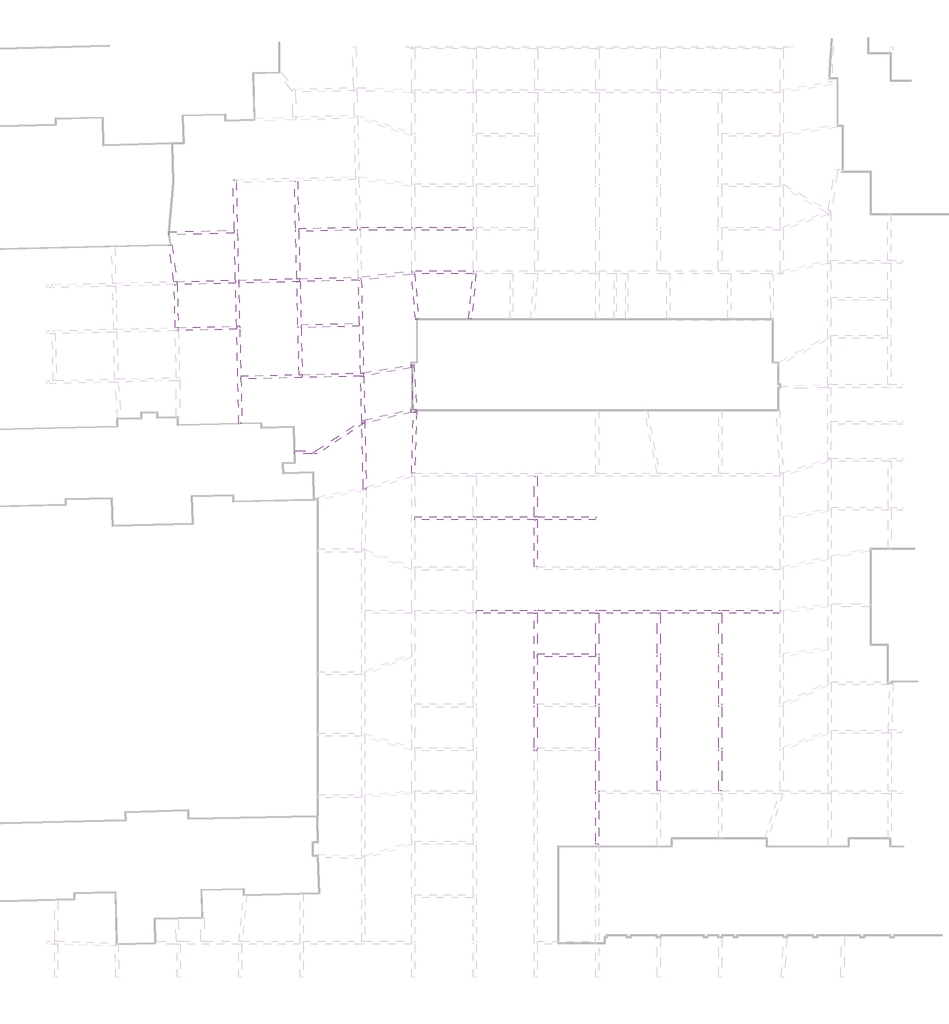
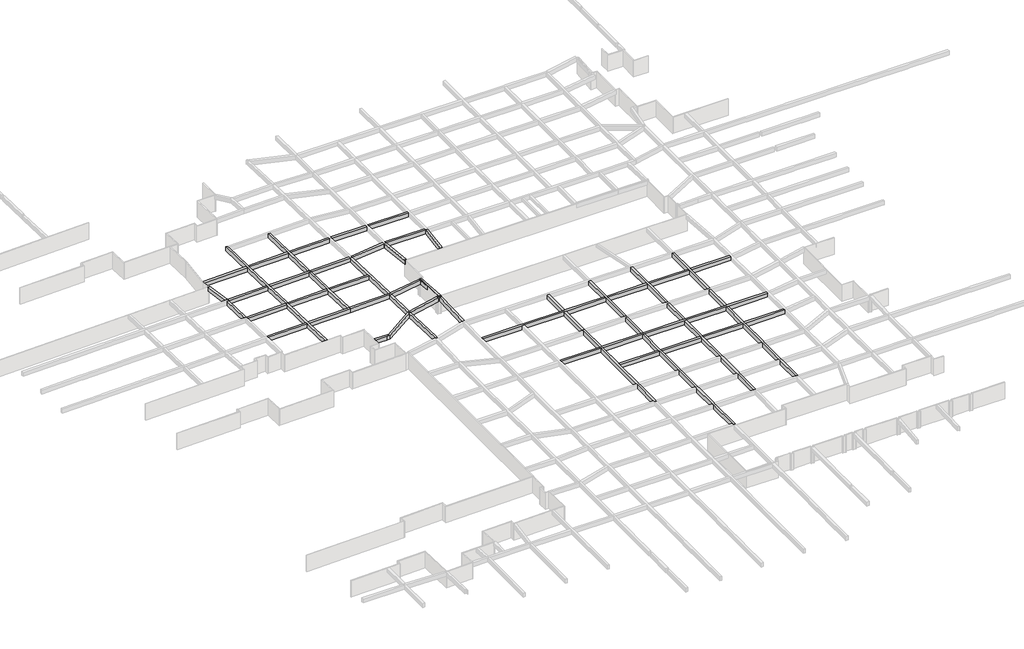
# One storey, part 11 of 20: 39 beams.
"""IFC4 building model written with IfcOpenShell, lengths in millimetres."""

from ifc_helpers import new_model, si_unit, frame, origin, place, context, project, spatial, polyline, outline, extrude, faceted_brep, element, save

model = new_model("IFC4")

# Units and contexts
model_context = context("Model", 3, world=origin())
ifc_project = project(units=[si_unit("LENGTHUNIT", "METRE", prefix="MILLI")], contexts=[model_context])

# Site, building, storey
site = spatial("IfcSite", under=ifc_project)
building = spatial("IfcBuilding", under=site)
storey = spatial("IfcBuildingStorey", under=building, Name="户型图", Elevation=0.0)

# Beams
placement = place(None, origin())
element("IfcBeam", 1, ObjectType="混凝土 - 矩形梁 : KL_beam", at=placement, inside=storey, context=model_context, shape_type="SweptSolid", body=[
    extrude(outline(polyline([(54450.0, 125765.1975441), (54450.0, 125365.1975441), (47756.2911881, 125365.1975441), (47746.6524387, 125765.1975441), (54450.0, 125765.1975441)])), frame((0.0, 0.0, 2500.0), z_axis=(0.0, 0.0, 1.0), x_axis=(1.0, 0.0, 0.0)), (0.0, 0.0, 1.0), 800.0),
])
element("IfcBeam", 2, ObjectType="混凝土 - 矩形梁 : KL_beam", at=placement, inside=storey, context=model_context, shape_type="SweptSolid", body=[
    extrude(outline(polyline([(62450.0, 125765.1975441), (62450.0, 125365.1975441), (54850.0, 125365.1975441), (54850.0, 125765.1975441), (62450.0, 125765.1975441)])), frame((0.0, 0.0, 2500.0), z_axis=(0.0, 0.0, 1.0), x_axis=(1.0, 0.0, 0.0)), (0.0, 0.0, 1.0), 800.0),
])
element("IfcBeam", 3, ObjectType="混凝土 - 矩形梁 : KL_beam", at=placement, inside=storey, context=model_context, shape_type="SweptSolid", body=[
    extrude(outline(polyline([(54450.0, 119664.8886593), (47912.3274647, 118889.8231887), (47902.648865, 119291.4769437), (54450.0, 120067.6898484), (54450.0, 119664.8886593)])), frame((0.0, 0.0, 2500.0), z_axis=(0.0, 0.0, 1.0), x_axis=(1.0, 0.0, 0.0)), (0.0, 0.0, 1.0), 800.0),
])
element("IfcBeam", 4, ObjectType="混凝土 - 矩形梁 : KL_beam", at=placement, inside=storey, context=model_context, shape_type="Brep", body=[
    faceted_brep([(62450.0, 119690.0, 3300.0), (62450.0, 120090.0, 3300.0), (54850.0, 120090.0, 3300.0), (54850.0, 119712.3101516, 3300.0), (54661.8140065, 119690.0, 3300.0), (54867.3687974, 119690.0, 3300.0), (62430.2407958, 119690.0, 3300.0), (62450.0, 119690.0, 2500.0), (54661.8140065, 119690.0, 2500.0), (54867.3687974, 119690.0, 2500.0), (62430.2407958, 119690.0, 2500.0), (62450.0, 120090.0, 2500.0), (54850.0, 119712.3101516, 2500.0), (54850.0, 120090.0, 2500.0)], [[[0, 1, 2, 3, 4, 5, 6]], [[7, 0, 6, 5, 4, 8, 9, 10]], [[11, 7, 10, 9, 8, 12, 13]], [[1, 11, 13, 2]], [[1, 0, 7, 11]], [[12, 3, 2, 13]], [[3, 12, 8, 4]]]),
])
element("IfcBeam", 5, ObjectType="混凝土 - 矩形梁 : KL_beam", at=placement, inside=storey, context=model_context, shape_type="Brep", body=[
    faceted_brep([(102445.0, 75460.0, 3300.0), (102445.0, 75860.0, 3300.0), (94850.0, 75860.0, 3300.0), (94450.0, 75860.0, 3300.0), (86850.0, 75860.0, 3300.0), (86450.0, 75860.0, 3300.0), (78850.0, 75860.0, 3300.0), (78450.0, 75860.0, 3300.0), (70850.0, 75860.0, 3300.0), (70450.0, 75860.0, 3300.0), (62850.0, 75860.0, 3300.0), (62850.0, 75460.0, 3300.0), (70450.0, 75460.0, 3300.0), (70850.0, 75460.0, 3300.0), (78450.0, 75460.0, 3300.0), (78850.0, 75460.0, 3300.0), (86450.0, 75460.0, 3300.0), (86850.0, 75460.0, 3300.0), (94450.0, 75460.0, 3300.0), (94850.0, 75460.0, 3300.0), (102445.0, 75460.0, 2500.0), (62850.0, 75460.0, 2500.0), (70450.0, 75460.0, 2500.0), (70850.0, 75460.0, 2500.0), (78450.0, 75460.0, 2500.0), (78850.0, 75460.0, 2500.0), (86450.0, 75460.0, 2500.0), (86850.0, 75460.0, 2500.0), (94450.0, 75460.0, 2500.0), (94850.0, 75460.0, 2500.0), (102445.0, 75860.0, 2500.0), (62850.0, 75860.0, 2500.0), (70450.0, 75860.0, 2500.0), (70850.0, 75860.0, 2500.0), (78450.0, 75860.0, 2500.0), (78850.0, 75860.0, 2500.0), (86450.0, 75860.0, 2500.0), (86850.0, 75860.0, 2500.0), (94450.0, 75860.0, 2500.0), (94850.0, 75860.0, 2500.0)], [[[0, 1, 2, 3, 4, 5, 6, 7, 8, 9, 10, 11, 12, 13, 14, 15, 16, 17, 18, 19]], [[20, 0, 19, 18, 17, 16, 15, 14, 13, 12, 11, 21, 22, 23, 24, 25, 26, 27, 28, 29]], [[30, 20, 29, 28, 27, 26, 25, 24, 23, 22, 21, 31, 32, 33, 34, 35, 36, 37, 38, 39]], [[1, 30, 39, 38, 37, 36, 35, 34, 33, 32, 31, 10, 9, 8, 7, 6, 5, 4, 3, 2]], [[1, 0, 20, 30]], [[11, 10, 31, 21]]]),
])
element("IfcBeam", 6, ObjectType="混凝土 - 矩形梁 : KL_beam", at=placement, inside=storey, context=model_context, shape_type="Brep", body=[
    faceted_brep([(70450.0, 57560.0, 3300.0), (70850.0, 57560.0, 3300.0), (70850.0, 57960.0, 3300.0), (70850.0, 63283.0, 3300.0), (70850.0, 63683.0, 3300.0), (70850.0, 69810.0, 3300.0), (70850.0, 70210.0, 3300.0), (70850.0, 75460.0, 3300.0), (70450.0, 75460.0, 3300.0), (70450.0, 63660.0, 3300.0), (70450.0, 63260.0, 3300.0), (70450.0, 57960.0, 3300.0), (70450.0, 57560.0, 2500.0), (70450.0, 75460.0, 2500.0), (70450.0, 63660.0, 2500.0), (70450.0, 63260.0, 2500.0), (70450.0, 57960.0, 2500.0), (70850.0, 57560.0, 2500.0), (70850.0, 75460.0, 2500.0), (70850.0, 70210.0, 2500.0), (70850.0, 69810.0, 2500.0), (70850.0, 63683.0, 2500.0), (70850.0, 63283.0, 2500.0), (70850.0, 57960.0, 2500.0)], [[[0, 1, 2, 3, 4, 5, 6, 7, 8, 9, 10, 11]], [[12, 0, 11, 10, 9, 8, 13, 14, 15, 16]], [[17, 12, 16, 15, 14, 13, 18, 19, 20, 21, 22, 23]], [[1, 17, 23, 22, 21, 20, 19, 18, 7, 6, 5, 4, 3, 2]], [[8, 7, 18, 13]], [[1, 0, 12, 17]]]),
    faceted_brep([(70850.0, 75860.0, 3300.0), (70450.0, 75860.0, 3300.0), (70450.0, 75860.0, 2500.0), (70850.0, 75860.0, 2500.0), (70850.0, 81560.0, 3300.0), (70450.0, 81560.0, 3300.0), (70450.0, 81510.0, 3300.0), (70450.0, 81110.0, 3300.0), (70850.0, 81160.0, 3300.0), (70450.0, 81560.0, 2500.0), (70450.0, 81510.0, 2500.0), (70450.0, 81110.0, 2500.0), (70850.0, 81560.0, 2500.0), (70850.0, 81160.0, 2500.0)], [[[0, 1, 2, 3]], [[4, 5, 6, 7, 1, 0, 8]], [[5, 9, 10, 11, 2, 1, 7, 6]], [[9, 12, 13, 3, 2, 11, 10]], [[12, 4, 8, 0, 3, 13]], [[5, 4, 12, 9]]]),
])
element("IfcBeam", 7, ObjectType="混凝土 - 矩形梁 : KL_beam", at=placement, inside=storey, context=model_context, shape_type="Brep", body=[
    faceted_brep([(78450.0, 81560.0, 3300.0), (78850.0, 81560.0, 3300.0), (78850.0, 87660.0, 3300.0), (78850.0, 88060.0, 3300.0), (78850.0, 93310.0, 3300.0), (78450.0, 93310.0, 3300.0), (78450.0, 88060.0, 3300.0), (78450.0, 87660.0, 3300.0), (78450.0, 81560.0, 2500.0), (78450.0, 93310.0, 2500.0), (78450.0, 88060.0, 2500.0), (78450.0, 87660.0, 2500.0), (78850.0, 81560.0, 2500.0), (78850.0, 93310.0, 2500.0), (78850.0, 88060.0, 2500.0), (78850.0, 87660.0, 2500.0)], [[[0, 1, 2, 3, 4, 5, 6, 7]], [[8, 0, 7, 6, 5, 9, 10, 11]], [[12, 8, 11, 10, 9, 13, 14, 15]], [[1, 12, 15, 14, 13, 4, 3, 2]], [[1, 0, 8, 12]], [[5, 4, 13, 9]]]),
    faceted_brep([(78450.0, 75460.0, 3300.0), (78850.0, 75460.0, 3300.0), (78850.0, 75460.0, 2500.0), (78450.0, 75460.0, 2500.0), (78450.0, 70210.0, 3300.0), (78450.0, 69810.0, 3300.0), (78450.0, 63683.0, 3300.0), (78450.0, 63283.0, 3300.0), (78450.0, 57960.0, 3300.0), (78450.0, 57560.0, 3300.0), (78450.0, 52365.0, 3300.0), (78450.0, 51965.0, 3300.0), (78450.0, 45760.0, 3300.0), (78450.0, 45360.0, 3300.0), (78850.0, 45360.0, 3300.0), (78850.0, 51965.0, 3300.0), (78850.0, 52365.0, 3300.0), (78850.0, 57560.0, 3300.0), (78850.0, 57960.0, 3300.0), (78850.0, 63283.0, 3300.0), (78850.0, 63683.0, 3300.0), (78850.0, 69810.0, 3300.0), (78850.0, 70210.0, 3300.0), (78450.0, 70210.0, 2500.0), (78450.0, 69810.0, 2500.0), (78450.0, 63683.0, 2500.0), (78450.0, 63283.0, 2500.0), (78450.0, 57960.0, 2500.0), (78450.0, 57560.0, 2500.0), (78450.0, 52365.0, 2500.0), (78450.0, 51965.0, 2500.0), (78450.0, 45760.0, 2500.0), (78450.0, 45360.0, 2500.0), (78850.0, 70210.0, 2500.0), (78850.0, 69810.0, 2500.0), (78850.0, 63683.0, 2500.0), (78850.0, 63283.0, 2500.0), (78850.0, 57960.0, 2500.0), (78850.0, 57560.0, 2500.0), (78850.0, 52365.0, 2500.0), (78850.0, 51965.0, 2500.0), (78850.0, 45360.0, 2500.0)], [[[0, 1, 2, 3]], [[1, 0, 4, 5, 6, 7, 8, 9, 10, 11, 12, 13, 14, 15, 16, 17, 18, 19, 20, 21, 22]], [[0, 3, 23, 24, 25, 26, 27, 28, 29, 30, 31, 32, 13, 12, 11, 10, 9, 8, 7, 6, 5, 4]], [[3, 2, 33, 34, 35, 36, 37, 38, 39, 40, 41, 32, 31, 30, 29, 28, 27, 26, 25, 24, 23]], [[2, 1, 22, 21, 20, 19, 18, 17, 16, 15, 14, 41, 40, 39, 38, 37, 36, 35, 34, 33]], [[14, 13, 32, 41]]]),
    faceted_brep([(78850.0, 75860.0, 3300.0), (78450.0, 75860.0, 3300.0), (78450.0, 75860.0, 2500.0), (78850.0, 75860.0, 2500.0), (78450.0, 81160.0, 3300.0), (78850.0, 81160.0, 3300.0), (78850.0, 81160.0, 2500.0), (78450.0, 81160.0, 2500.0)], [[[0, 1, 2, 3]], [[4, 5, 6, 7]], [[1, 0, 5, 4]], [[2, 1, 4, 7]], [[3, 2, 7, 6]], [[0, 3, 6, 5]]]),
])
element("IfcBeam", 8, ObjectType="混凝土 - 矩形梁 : KL_beam", at=placement, inside=storey, context=model_context, shape_type="Brep", body=[
    faceted_brep([(86450.0, 81560.0, 3300.0), (86850.0, 81560.0, 3300.0), (86850.0, 87660.0, 3300.0), (86850.0, 88060.0, 3300.0), (86850.0, 93310.0, 3300.0), (86450.0, 93310.0, 3300.0), (86450.0, 88060.0, 3300.0), (86450.0, 87660.0, 3300.0), (86450.0, 81560.0, 2500.0), (86450.0, 93310.0, 2500.0), (86450.0, 88060.0, 2500.0), (86450.0, 87660.0, 2500.0), (86850.0, 81560.0, 2500.0), (86850.0, 93310.0, 2500.0), (86850.0, 88060.0, 2500.0), (86850.0, 87660.0, 2500.0)], [[[0, 1, 2, 3, 4, 5, 6, 7]], [[8, 0, 7, 6, 5, 9, 10, 11]], [[12, 8, 11, 10, 9, 13, 14, 15]], [[1, 12, 15, 14, 13, 4, 3, 2]], [[1, 0, 8, 12]], [[5, 4, 13, 9]]]),
    faceted_brep([(86450.0, 75460.0, 3300.0), (86850.0, 75460.0, 3300.0), (86850.0, 75460.0, 2500.0), (86450.0, 75460.0, 2500.0), (86450.0, 70210.0, 3300.0), (86450.0, 69810.0, 3300.0), (86450.0, 63683.0, 3300.0), (86450.0, 63283.0, 3300.0), (86450.0, 57960.0, 3300.0), (86450.0, 57560.0, 3300.0), (86450.0, 52365.0, 3300.0), (86850.0, 52365.0, 3300.0), (86850.0, 57560.0, 3300.0), (86850.0, 57960.0, 3300.0), (86850.0, 63283.0, 3300.0), (86850.0, 63683.0, 3300.0), (86850.0, 69810.0, 3300.0), (86850.0, 70210.0, 3300.0), (86450.0, 70210.0, 2500.0), (86450.0, 69810.0, 2500.0), (86450.0, 63683.0, 2500.0), (86450.0, 63283.0, 2500.0), (86450.0, 57960.0, 2500.0), (86450.0, 57560.0, 2500.0), (86450.0, 52365.0, 2500.0), (86850.0, 70210.0, 2500.0), (86850.0, 69810.0, 2500.0), (86850.0, 63683.0, 2500.0), (86850.0, 63283.0, 2500.0), (86850.0, 57960.0, 2500.0), (86850.0, 57560.0, 2500.0), (86850.0, 52365.0, 2500.0)], [[[0, 1, 2, 3]], [[1, 0, 4, 5, 6, 7, 8, 9, 10, 11, 12, 13, 14, 15, 16, 17]], [[0, 3, 18, 19, 20, 21, 22, 23, 24, 10, 9, 8, 7, 6, 5, 4]], [[3, 2, 25, 26, 27, 28, 29, 30, 31, 24, 23, 22, 21, 20, 19, 18]], [[2, 1, 17, 16, 15, 14, 13, 12, 11, 31, 30, 29, 28, 27, 26, 25]], [[11, 10, 24, 31]]]),
    faceted_brep([(86850.0, 75860.0, 3300.0), (86450.0, 75860.0, 3300.0), (86450.0, 75860.0, 2500.0), (86850.0, 75860.0, 2500.0), (86450.0, 81160.0, 3300.0), (86850.0, 81160.0, 3300.0), (86850.0, 81160.0, 2500.0), (86450.0, 81160.0, 2500.0)], [[[0, 1, 2, 3]], [[4, 5, 6, 7]], [[1, 0, 5, 4]], [[2, 1, 4, 7]], [[3, 2, 7, 6]], [[0, 3, 6, 5]]]),
])
element("IfcBeam", 9, ObjectType="混凝土 - 矩形梁 : KL_beam", at=placement, inside=storey, context=model_context, shape_type="Brep", body=[
    faceted_brep([(94850.0, 75460.0, 3300.0), (94450.0, 75460.0, 3300.0), (94450.0, 70210.0, 3300.0), (94450.0, 69810.0, 3300.0), (94450.0, 63683.0, 3300.0), (94450.0, 63283.0, 3300.0), (94450.0, 57960.0, 3300.0), (94450.0, 57560.0, 3300.0), (94450.0, 52365.0, 3300.0), (94850.0, 52365.0, 3300.0), (94850.0, 57560.0, 3300.0), (94850.0, 57960.0, 3300.0), (94850.0, 63283.0, 3300.0), (94850.0, 63683.0, 3300.0), (94850.0, 69810.0, 3300.0), (94850.0, 70210.0, 3300.0), (94850.0, 75460.0, 2500.0), (94850.0, 52365.0, 2500.0), (94850.0, 57560.0, 2500.0), (94850.0, 57960.0, 2500.0), (94850.0, 63283.0, 2500.0), (94850.0, 63683.0, 2500.0), (94850.0, 69810.0, 2500.0), (94850.0, 70210.0, 2500.0), (94450.0, 75460.0, 2500.0), (94450.0, 52365.0, 2500.0), (94450.0, 57560.0, 2500.0), (94450.0, 57960.0, 2500.0), (94450.0, 63283.0, 2500.0), (94450.0, 63683.0, 2500.0), (94450.0, 69810.0, 2500.0), (94450.0, 70210.0, 2500.0)], [[[0, 1, 2, 3, 4, 5, 6, 7, 8, 9, 10, 11, 12, 13, 14, 15]], [[16, 0, 15, 14, 13, 12, 11, 10, 9, 17, 18, 19, 20, 21, 22, 23]], [[24, 16, 23, 22, 21, 20, 19, 18, 17, 25, 26, 27, 28, 29, 30, 31]], [[1, 24, 31, 30, 29, 28, 27, 26, 25, 8, 7, 6, 5, 4, 3, 2]], [[1, 0, 16, 24]], [[9, 8, 25, 17]]]),
    faceted_brep([(94850.0, 75860.0, 3300.0), (94450.0, 75860.0, 3300.0), (94450.0, 75860.0, 2500.0), (94850.0, 75860.0, 2500.0), (94450.0, 81160.0, 3300.0), (94850.0, 81160.0, 3300.0), (94850.0, 81160.0, 2500.0), (94450.0, 81160.0, 2500.0)], [[[0, 1, 2, 3]], [[4, 5, 6, 7]], [[1, 0, 5, 4]], [[0, 3, 6, 5]], [[3, 2, 7, 6]], [[2, 1, 4, 7]]]),
    faceted_brep([(94450.0, 81560.0, 3300.0), (94850.0, 81560.0, 3300.0), (94850.0, 87660.0, 3300.0), (94850.0, 88060.0, 3300.0), (94850.0, 93310.0, 3300.0), (94450.0, 93310.0, 3300.0), (94450.0, 88060.0, 3300.0), (94450.0, 87660.0, 3300.0), (94850.0, 81560.0, 2500.0), (94850.0, 87660.0, 2500.0), (94850.0, 88060.0, 2500.0), (94850.0, 93310.0, 2500.0), (94450.0, 81560.0, 2500.0), (94450.0, 87660.0, 2500.0), (94450.0, 88060.0, 2500.0), (94450.0, 93310.0, 2500.0)], [[[0, 1, 2, 3, 4, 5, 6, 7]], [[1, 8, 9, 10, 11, 4, 3, 2]], [[8, 12, 13, 14, 15, 11, 10, 9]], [[12, 0, 7, 6, 5, 15, 14, 13]], [[1, 0, 12, 8]], [[5, 4, 11, 15]]]),
])
element("IfcBeam", 10, ObjectType="混凝土 - 矩形梁 : KL_beam", at=placement, inside=storey, context=model_context, shape_type="Brep", body=[
    faceted_brep([(78450.0, 87660.0, 3300.0), (78450.0, 88060.0, 3300.0), (70850.0, 88060.0, 3300.0), (70450.0, 88060.0, 3300.0), (62850.0, 88060.0, 3300.0), (62450.0, 88060.0, 3300.0), (54850.0, 88060.0, 3300.0), (54850.0, 87660.0, 3300.0), (62450.0, 87660.0, 3300.0), (62850.0, 87660.0, 3300.0), (70450.0, 87660.0, 3300.0), (70850.0, 87660.0, 3300.0), (78450.0, 87660.0, 2500.0), (54850.0, 87660.0, 2500.0), (62450.0, 87660.0, 2500.0), (62850.0, 87660.0, 2500.0), (70450.0, 87660.0, 2500.0), (70850.0, 87660.0, 2500.0), (78450.0, 88060.0, 2500.0), (54850.0, 88060.0, 2500.0), (62450.0, 88060.0, 2500.0), (62850.0, 88060.0, 2500.0), (70450.0, 88060.0, 2500.0), (70850.0, 88060.0, 2500.0)], [[[0, 1, 2, 3, 4, 5, 6, 7, 8, 9, 10, 11]], [[12, 0, 11, 10, 9, 8, 7, 13, 14, 15, 16, 17]], [[18, 12, 17, 16, 15, 14, 13, 19, 20, 21, 22, 23]], [[1, 18, 23, 22, 21, 20, 19, 6, 5, 4, 3, 2]], [[1, 0, 12, 18]], [[7, 6, 19, 13]]]),
    faceted_brep([(102445.0, 88060.0, 3300.0), (102445.0, 87660.0, 3300.0), (102445.0, 87660.0, 2500.0), (102445.0, 88060.0, 2500.0), (94850.0, 87660.0, 3300.0), (94850.0, 88060.0, 3300.0), (94850.0, 88060.0, 2500.0), (94850.0, 87660.0, 2500.0)], [[[0, 1, 2, 3]], [[4, 5, 6, 7]], [[1, 0, 5, 4]], [[2, 1, 4, 7]], [[3, 2, 7, 6]], [[0, 3, 6, 5]]]),
    faceted_brep([(78850.0, 87660.0, 3300.0), (78850.0, 88060.0, 3300.0), (78850.0, 88060.0, 2500.0), (78850.0, 87660.0, 2500.0), (86450.0, 88060.0, 3300.0), (86450.0, 87660.0, 3300.0), (86450.0, 87660.0, 2500.0), (86450.0, 88060.0, 2500.0)], [[[0, 1, 2, 3]], [[4, 5, 6, 7]], [[1, 0, 5, 4]], [[0, 3, 6, 5]], [[3, 2, 7, 6]], [[2, 1, 4, 7]]]),
    faceted_brep([(86850.0, 88060.0, 3300.0), (86850.0, 87660.0, 3300.0), (94450.0, 87660.0, 3300.0), (94450.0, 88060.0, 3300.0), (86850.0, 87660.0, 2500.0), (94450.0, 87660.0, 2500.0), (86850.0, 88060.0, 2500.0), (94450.0, 88060.0, 2500.0)], [[[0, 1, 2, 3]], [[1, 4, 5, 2]], [[4, 6, 7, 5]], [[6, 0, 3, 7]], [[1, 0, 6, 4]], [[3, 2, 5, 7]]]),
])
element("IfcBeam", 11, ObjectType="混凝土 - 矩形梁 : KL_beam", at=placement, inside=storey, context=model_context, shape_type="SweptSolid", body=[
    extrude(outline(polyline([(102445.0, 70210.0), (102445.0, 69810.0), (94850.0, 69810.0), (94850.0, 70210.0), (102445.0, 70210.0)])), frame((0.0, 0.0, 2500.0), z_axis=(0.0, 0.0, 1.0), x_axis=(1.0, 0.0, 0.0)), (0.0, 0.0, 1.0), 800.0),
    extrude(outline(polyline([(70850.0, 69810.0), (70850.0, 70210.0), (78450.0, 70210.0), (78450.0, 69810.0), (70850.0, 69810.0)])), frame((0.0, 0.0, 2500.0), z_axis=(0.0, 0.0, 1.0), x_axis=(1.0, 0.0, 0.0)), (0.0, 0.0, 1.0), 800.0),
    extrude(outline(polyline([(78850.0, 69810.0), (78850.0, 70210.0), (86450.0, 70210.0), (86450.0, 69810.0), (78850.0, 69810.0)])), frame((0.0, 0.0, 2500.0), z_axis=(0.0, 0.0, 1.0), x_axis=(1.0, 0.0, 0.0)), (0.0, 0.0, 1.0), 800.0),
    extrude(outline(polyline([(86850.0, 69810.0), (86850.0, 70210.0), (94450.0, 70210.0), (94450.0, 69810.0), (86850.0, 69810.0)])), frame((0.0, 0.0, 2500.0), z_axis=(0.0, 0.0, 1.0), x_axis=(1.0, 0.0, 0.0)), (0.0, 0.0, 1.0), 800.0),
])
element("IfcBeam", 12, ObjectType="混凝土 - 矩形梁 : KL_beam", at=placement, inside=storey, context=model_context, shape_type="SweptSolid", body=[
    extrude(outline(polyline([(70450.0, 93310.0), (70850.0, 93310.0), (70850.0, 88060.0), (70450.0, 88060.0), (70450.0, 93310.0)])), frame((0.0, 0.0, 2500.0), z_axis=(0.0, 0.0, 1.0), x_axis=(1.0, 0.0, 0.0)), (0.0, 0.0, 1.0), 800.0),
])
element("IfcBeam", 13, ObjectType="混凝土 - 矩形梁 : KL_beam", at=placement, inside=storey, context=model_context, shape_type="SweptSolid", body=[
    extrude(outline(polyline([(70850.0, 81560.0), (70450.0, 81560.0), (70450.0, 87660.0), (70850.0, 87660.0), (70850.0, 81560.0)])), frame((0.0, 0.0, 2500.0), z_axis=(0.0, 0.0, 1.0), x_axis=(1.0, 0.0, 0.0)), (0.0, 0.0, 1.0), 800.0),
])
element("IfcBeam", 14, ObjectType="混凝土 - 矩形梁 : KL_beam", at=placement, inside=storey, context=model_context, shape_type="Brep", body=[
    faceted_brep([(61879.8710047, 113857.0, 3300.0), (62281.6476136, 113857.0, 3300.0), (62832.0174047, 119690.0, 3300.0), (62450.0, 119690.0, 3300.0), (62430.2407958, 119690.0, 3300.0), (61879.8710047, 113857.0, 2500.0), (62430.2407958, 119690.0, 2500.0), (62281.6476136, 113857.0, 2500.0), (62450.0, 119690.0, 2500.0), (62832.0174047, 119690.0, 2500.0)], [[[0, 1, 2, 3, 4]], [[5, 0, 4, 6]], [[7, 5, 6, 8, 9]], [[1, 7, 9, 2]], [[1, 0, 5, 7]], [[2, 9, 8, 6, 4, 3]]]),
])
element("IfcBeam", 15, ObjectType="混凝土 - 矩形梁 : KL_beam", at=placement, inside=storey, context=model_context, shape_type="SweptSolid", body=[
    extrude(outline(polyline([(55098.0, 113737.0), (54962.3085372, 113737.0), (54467.8976834, 119667.0104964), (54661.8140065, 119690.0), (54867.3687974, 119690.0), (55353.6914628, 113857.0), (55098.0, 113857.0), (55098.0, 113737.0)])), frame((0.0, 0.0, 2500.0), z_axis=(0.0, 0.0, 1.0), x_axis=(1.0, 0.0, 0.0)), (0.0, 0.0, 1.0), 800.0),
])
element("IfcBeam", 16, ObjectType="混凝土 - 矩形梁 : KL_beam", at=placement, inside=storey, context=model_context, shape_type="SweptSolid", body=[
    extrude(outline(polyline([(22839.9092142, 123427.099828), (23236.2427496, 123481.1343421), (23889.0031982, 118693.2527351), (23486.6252708, 118683.5527596), (22839.9092142, 123427.099828)])), frame((0.0, 0.0, 2500.0), z_axis=(0.0, 0.0, 1.0), x_axis=(1.0, 0.0, 0.0)), (0.0, 0.0, 1.0), 800.0),
])
element("IfcBeam", 17, ObjectType="混凝土 - 矩形梁 : KL_beam", at=placement, inside=storey, context=model_context, shape_type="Brep", body=[
    faceted_brep([(23889.0031982, 118693.2527351, 3300.0), (23898.6430493, 118293.3689104, 3300.0), (23540.9968018, 118284.7472649, 3300.0), (23519.8781337, 118284.238165, 3300.0), (23654.8569706, 112685.136784, 3300.0), (24054.7407895, 112694.7768761, 3300.0), (23919.7618713, 118293.8816298, 3300.0), (23910.1218663, 118693.761835, 3300.0), (23519.8781337, 118284.238165, 2500.0), (23654.8569706, 112685.136784, 2500.0), (23898.6430493, 118293.3689104, 2500.0), (23889.0031982, 118693.2527351, 2500.0), (23910.1218663, 118693.761835, 2500.0), (23919.7618713, 118293.8816298, 2500.0), (24054.7407895, 112694.7768761, 2500.0), (23540.9968018, 118284.7472649, 2500.0)], [[[0, 1, 2, 3, 4, 5, 6, 7]], [[3, 8, 9, 4]], [[10, 11, 12, 13, 14, 9, 8, 15]], [[12, 7, 6, 5, 14, 13]], [[11, 0, 7, 12]], [[1, 10, 15, 8, 3, 2]], [[10, 1, 0, 11]], [[5, 4, 9, 14]]]),
])
element("IfcBeam", 18, ObjectType="混凝土 - 矩形梁 : KL_beam", at=placement, inside=storey, context=model_context, shape_type="Brep", body=[
    faceted_brep([(32052.1182859, 112886.7653645, 3300.0), (31652.2346355, 112877.1182859, 3300.0), (31661.8588222, 112478.1835343, 3300.0), (31956.7693302, 100253.7688116, 3300.0), (32356.6529807, 100263.4158903, 3300.0), (32218.5158115, 105989.3768117, 3300.0), (32208.8687328, 106389.2604627, 3300.0), (32061.7653645, 112486.8817141, 3300.0), (31652.2346355, 112877.1182859, 2500.0), (31661.8588222, 112478.1835343, 2500.0), (31956.7693302, 100253.7688116, 2500.0), (32052.1182859, 112886.7653645, 2500.0), (32061.7653645, 112486.8817141, 2500.0), (32208.8687328, 106389.2604627, 2500.0), (32218.5158115, 105989.3768117, 2500.0), (32356.6529807, 100263.4158903, 2500.0)], [[[0, 1, 2, 3, 4, 5, 6, 7]], [[1, 8, 9, 10, 3, 2]], [[8, 11, 12, 13, 14, 15, 10, 9]], [[11, 0, 7, 6, 5, 4, 15, 14, 13, 12]], [[4, 3, 10, 15]], [[1, 0, 11, 8]]]),
])
element("IfcBeam", 19, ObjectType="混凝土 - 矩形梁 : KL_beam", at=placement, inside=storey, context=model_context, shape_type="Brep", body=[
    faceted_brep([(24216.2679247, 105994.416832, 3300.0), (24221.0300595, 105796.8771597, 3300.0), (31818.6316338, 105979.7515911, 3300.0), (31808.9845551, 106379.6352421, 3300.0), (24216.2679247, 106196.8783914, 3300.0), (24221.0300595, 105796.8771597, 2500.0), (31818.6316338, 105979.7515911, 2500.0), (24216.2679247, 105994.416832, 2500.0), (24216.2679247, 106196.8783914, 2500.0), (31808.9845551, 106379.6352421, 2500.0)], [[[0, 1, 2, 3, 4]], [[1, 5, 6, 2]], [[5, 7, 8, 9, 6]], [[8, 4, 3, 9]], [[5, 1, 0, 7]], [[0, 4, 8, 7]], [[3, 2, 6, 9]]]),
    faceted_brep([(32218.5158115, 105989.3768117, 3300.0), (32208.8687328, 106389.2604627, 3300.0), (32208.8687328, 106389.2604627, 2500.0), (32218.5158115, 105989.3768117, 2500.0), (40215.5578613, 106181.8657839, 3300.0), (40205.9326406, 106581.749961, 3300.0), (39806.0484635, 106572.1247404, 3300.0), (40215.5578613, 106181.8657839, 2500.0), (40205.9326406, 106581.749961, 2500.0), (39806.0484635, 106572.1247404, 2500.0)], [[[0, 1, 2, 3]], [[4, 5, 6, 1, 0]], [[7, 4, 0, 3]], [[8, 7, 3, 2, 9]], [[5, 8, 9, 2, 1, 6]], [[5, 4, 7, 8]]]),
])
element("IfcBeam", 20, ObjectType="混凝土 - 矩形梁 : KL_beam", at=placement, inside=storey, context=model_context, shape_type="Brep", body=[
    faceted_brep([(40205.9323475, 106581.7621411, 3300.0), (40215.5575681, 106181.8779632, 3300.0), (47814.3531628, 106365.2447486, 3300.0), (48028.6784416, 106370.4166389, 3300.0), (48214.331784, 106374.8966458, 3300.0), (48213.6881872, 106401.5675651, 3300.0), (48204.68218, 106774.7802353, 3300.0), (47804.7985905, 106765.1306313, 3300.0), (40215.5575681, 106181.8779632, 2500.0), (47814.3531628, 106365.2447486, 2500.0), (48028.6784416, 106370.4166389, 2500.0), (48214.331784, 106374.8966458, 2500.0), (40205.9323475, 106581.7621411, 2500.0), (47804.7985905, 106765.1306313, 2500.0), (48204.68218, 106774.7802353, 2500.0), (48213.6881872, 106401.5675651, 2500.0)], [[[0, 1, 2, 3, 4, 5, 6, 7]], [[1, 8, 9, 10, 11, 4, 3, 2]], [[8, 12, 13, 14, 15, 11, 10, 9]], [[12, 0, 7, 6, 14, 13]], [[1, 0, 12, 8]], [[6, 5, 4, 11, 15, 14]]]),
])
element("IfcBeam", 21, ObjectType="混凝土 - 矩形梁 : KL_beam", at=placement, inside=storey, context=model_context, shape_type="Brep", body=[
    faceted_brep([(39914.7549851, 118678.8583282, 3300.0), (39914.7479902, 118679.1489348, 3300.0), (39905.1297644, 119078.7425061, 3300.0), (31907.3709933, 118886.7242888, 3300.0), (31917.018072, 118486.8406357, 3300.0), (39914.7549851, 118678.8583282, 2500.0), (31917.018072, 118486.8406357, 2500.0), (39905.1297644, 119078.7425061, 2500.0), (39914.7479902, 118679.1489348, 2500.0), (31907.3709933, 118886.7242888, 2500.0)], [[[0, 1, 2, 3, 4]], [[5, 0, 4, 6]], [[7, 8, 5, 6, 9]], [[2, 7, 9, 3]], [[2, 1, 0, 5, 8, 7]], [[4, 3, 9, 6]]]),
])
element("IfcBeam", 22, ObjectType="混凝土 - 矩形梁 : KL_beam", at=placement, inside=storey, context=model_context, shape_type="Brep", body=[
    faceted_brep([(47912.3274647, 118889.8231887, 3300.0), (47512.443546, 118880.1872365, 3300.0), (47503.6725353, 119244.1768113, 3300.0), (47503.2400646, 119262.1239832, 3300.0), (39903.9405782, 119079.004625, 3300.0), (39504.056658, 119069.3686727, 3300.0), (39504.0627895, 119069.1132877, 3300.0), (39505.2450003, 119069.1416714, 3300.0), (39905.1297644, 119078.7425061, 3300.0), (39914.7479902, 118679.1489348, 3300.0), (47512.8828425, 118862.240229, 3300.0), (47912.7599354, 118871.8760168, 3300.0), (47503.2400646, 119262.1239832, 2500.0), (39903.9405782, 119079.004625, 2500.0), (39504.056658, 119069.3686727, 2500.0), (47512.443546, 118880.1872365, 2500.0), (47912.3274647, 118889.8231887, 2500.0), (47912.7599354, 118871.8760168, 2500.0), (47512.8828425, 118862.240229, 2500.0), (39914.7479902, 118679.1489348, 2500.0), (39905.1297644, 119078.7425061, 2500.0), (39505.2450003, 119069.1416714, 2500.0), (39504.0627895, 119069.1132877, 2500.0), (47503.6725353, 119244.1768113, 2500.0)], [[[0, 1, 2, 3, 4, 5, 6, 7, 8, 9, 10, 11]], [[3, 12, 13, 14, 5, 4]], [[15, 16, 17, 18, 19, 20, 21, 22, 14, 13, 12, 23]], [[11, 10, 9, 19, 18, 17]], [[16, 0, 11, 17]], [[1, 15, 23, 12, 3, 2]], [[15, 1, 0, 16]], [[20, 8, 7, 6, 22, 21]], [[8, 20, 19, 9]], [[5, 14, 22, 6]]]),
])
element("IfcBeam", 23, ObjectType="混凝土 - 矩形梁 : KL_beam", at=placement, inside=storey, context=model_context, shape_type="Brep", body=[
    faceted_brep([(39806.0484635, 106572.1247404, 3300.0), (40205.9326406, 106581.749961, 3300.0), (40059.1520523, 112679.8163801, 3300.0), (40049.5268316, 113079.7005578, 3300.0), (39914.7549851, 118678.8583282, 3300.0), (39514.8702209, 118669.2574936, 3300.0), (39649.6431806, 113070.0534791, 3300.0), (39659.2684013, 112670.1693014, 3300.0), (39806.0484635, 106572.1247404, 2500.0), (39514.8702209, 118669.2574936, 2500.0), (39649.6431806, 113070.0534791, 2500.0), (39659.2684013, 112670.1693014, 2500.0), (40205.9326406, 106581.749961, 2500.0), (39914.7549851, 118678.8583282, 2500.0), (40049.5268316, 113079.7005578, 2500.0), (40059.1520523, 112679.8163801, 2500.0)], [[[0, 1, 2, 3, 4, 5, 6, 7]], [[8, 0, 7, 6, 5, 9, 10, 11]], [[12, 8, 11, 10, 9, 13, 14, 15]], [[1, 12, 15, 14, 13, 4, 3, 2]], [[1, 0, 8, 12]], [[5, 4, 13, 9]]]),
])
element("IfcBeam", 24, ObjectType="混凝土 - 矩形梁 : KL_beam", at=placement, inside=storey, context=model_context, shape_type="SweptSolid", body=[
    extrude(outline(polyline([(40059.1520523, 112679.8163801), (40049.5268316, 113079.7005578), (47647.9980144, 113263.0115013), (47657.6476184, 112863.1279118), (40059.1520523, 112679.8163801)])), frame((0.0, 0.0, 2500.0), z_axis=(0.0, 0.0, 1.0), x_axis=(1.0, 0.0, 0.0)), (0.0, 0.0, 1.0), 800.0),
    extrude(outline(polyline([(32061.7653645, 112486.8817141), (32052.1182859, 112886.7653645), (39649.6431806, 113070.0534791), (39659.2684013, 112670.1693014), (32061.7653645, 112486.8817141)])), frame((0.0, 0.0, 2500.0), z_axis=(0.0, 0.0, 1.0), x_axis=(1.0, 0.0, 0.0)), (0.0, 0.0, 1.0), 800.0),
])
element("IfcBeam", 25, ObjectType="混凝土 - 矩形梁 : KL_beam", at=placement, inside=storey, context=model_context, shape_type="Brep", body=[
    faceted_brep([(47912.7667615, 118871.8761812, 3300.0), (47512.8828425, 118862.240229, 3300.0), (47647.9980144, 113263.0115013, 3300.0), (47657.6476184, 112863.1279118, 3300.0), (47804.7985905, 106765.1306313, 3300.0), (48204.68218, 106774.7802353, 3300.0), (48203.9395168, 106805.5565066, 3300.0), (47512.8828425, 118862.240229, 2500.0), (47647.9980144, 113263.0115013, 2500.0), (47657.6476184, 112863.1279118, 2500.0), (47804.7985905, 106765.1306313, 2500.0), (47912.7667615, 118871.8761812, 2500.0), (48203.9395168, 106805.5565066, 2500.0), (48204.68218, 106774.7802353, 2500.0)], [[[0, 1, 2, 3, 4, 5, 6]], [[1, 7, 8, 9, 10, 4, 3, 2]], [[7, 11, 12, 13, 10, 9, 8]], [[11, 0, 6, 5, 13, 12]], [[1, 0, 11, 7]], [[5, 4, 10, 13]]]),
])
element("IfcBeam", 26, ObjectType="混凝土 - 矩形梁 : KL_beam", at=placement, inside=storey, context=model_context, shape_type="Brep", body=[
    faceted_brep([(54340.0, 107586.0, 3300.0), (54340.0, 107838.7127137, 3300.0), (48203.9395168, 106805.5565066, 3300.0), (48204.68218, 106774.7802353, 3300.0), (48213.6881872, 106401.5675651, 3300.0), (54370.1111854, 107438.1523008, 3300.0), (54460.0, 107453.2872863, 3300.0), (54460.0, 107586.0, 3300.0), (54460.0, 107453.2872863, 2500.0), (48213.6881872, 106401.5675651, 2500.0), (54370.1111854, 107438.1523008, 2500.0), (54340.0, 107838.7127137, 2500.0), (54340.0, 107586.0, 2500.0), (54460.0, 107586.0, 2500.0), (48204.68218, 106774.7802353, 2500.0), (48203.9395168, 106805.5565066, 2500.0)], [[[0, 1, 2, 3, 4, 5, 6, 7]], [[8, 6, 5, 4, 9, 10]], [[11, 12, 13, 8, 10, 9, 14, 15]], [[1, 11, 15, 2]], [[6, 8, 13, 7]], [[0, 12, 11, 1]], [[9, 4, 3, 2, 15, 14]], [[12, 0, 7, 13]]]),
    faceted_brep([(47815.0815743, 106334.45237, 2500.0), (47815.0815743, 106334.45237, 3300.0), (47814.3531628, 106365.2447486, 3300.0), (47814.3531628, 106365.2447486, 2500.0), (48028.6784416, 106370.4166389, 3300.0), (48028.6784416, 106370.4166389, 2500.0)], [[[0, 1, 2, 3]], [[2, 4, 5, 3]], [[1, 4, 2]], [[1, 0, 5, 4]], [[5, 0, 3]]]),
])
element("IfcBeam", 27, ObjectType="混凝土 - 矩形梁 : KL_beam", at=placement, inside=storey, context=model_context, shape_type="Brep", body=[
    faceted_brep([(31652.2346355, 112877.1182859, 3300.0), (32052.1182859, 112886.7653645, 3300.0), (31759.2879616, 125024.9538327, 3300.0), (31749.6408829, 125424.8374833, 3300.0), (31601.1044653, 131581.8604473, 3300.0), (31591.4573866, 131981.7440979, 3300.0), (31191.5734678, 131972.1081457, 3300.0), (31350.6380438, 125378.6796589, 3300.0), (31360.2851224, 124978.7960085, 3300.0), (31507.4880057, 118877.0497356, 3300.0), (31517.1350844, 118477.1660852, 3300.0), (31652.2117435, 112878.0671847, 3300.0), (32052.1182859, 112886.7653645, 2500.0), (31759.2879616, 125024.9538327, 2500.0), (31749.6408829, 125424.8374833, 2500.0), (31601.1044653, 131581.8604473, 2500.0), (31591.4573866, 131981.7440979, 2500.0), (31652.2346355, 112877.1182859, 2500.0), (31652.2117435, 112878.0671847, 2500.0), (31517.1350844, 118477.1660852, 2500.0), (31507.4880057, 118877.0497356, 2500.0), (31360.2851224, 124978.7960085, 2500.0), (31350.6380438, 125378.6796589, 2500.0), (31191.5734678, 131972.1081457, 2500.0)], [[[0, 1, 2, 3, 4, 5, 6, 7, 8, 9, 10, 11]], [[1, 12, 13, 14, 15, 16, 5, 4, 3, 2]], [[12, 17, 18, 19, 20, 21, 22, 23, 16, 15, 14, 13]], [[17, 0, 11, 10, 9, 8, 7, 6, 23, 22, 21, 20, 19, 18]], [[1, 0, 17, 12]], [[6, 5, 16, 23]]]),
])
element("IfcBeam", 28, ObjectType="混凝土 - 矩形梁 : KL_beam", at=placement, inside=storey, context=model_context, shape_type="Brep", body=[
    faceted_brep([(39504.056658, 119069.3686727, 3300.0), (39903.9405782, 119079.004625, 3300.0), (39756.5575079, 125217.6630252, 3300.0), (39746.9566733, 125617.5477901, 3300.0), (39599.1322762, 131774.5879116, 3300.0), (39199.248356, 131764.9519594, 3300.0), (39347.072753, 125607.9118379, 3300.0), (39356.6735877, 125208.027073, 3300.0), (39504.056658, 119069.3686727, 2500.0), (39199.248356, 131764.9519594, 2500.0), (39347.072753, 125607.9118379, 2500.0), (39356.6735877, 125208.027073, 2500.0), (39903.9405782, 119079.004625, 2500.0), (39599.1322762, 131774.5879116, 2500.0), (39746.9566733, 125617.5477901, 2500.0), (39756.5575079, 125217.6630252, 2500.0)], [[[0, 1, 2, 3, 4, 5, 6, 7]], [[8, 0, 7, 6, 5, 9, 10, 11]], [[12, 8, 11, 10, 9, 13, 14, 15]], [[1, 12, 15, 14, 13, 4, 3, 2]], [[1, 0, 8, 12]], [[5, 4, 13, 9]]]),
])
element("IfcBeam", 29, ObjectType="混凝土 - 矩形梁 : KL_beam", at=placement, inside=storey, context=model_context, shape_type="SweptSolid", body=[
    extrude(outline(polyline([(47345.6819506, 125800.6533117), (47355.3179028, 125400.7693931), (39756.5575079, 125217.6630252), (39746.9566733, 125617.5477901), (47345.6819506, 125800.6533117)])), frame((0.0, 0.0, 2500.0), z_axis=(0.0, 0.0, 1.0), x_axis=(1.0, 0.0, 0.0)), (0.0, 0.0, 1.0), 800.0),
    extrude(outline(polyline([(31759.2879616, 125024.9538327), (31749.6408829, 125424.8374833), (39347.072753, 125607.9118379), (39356.6735877, 125208.027073), (31759.2879616, 125024.9538327)])), frame((0.0, 0.0, 2500.0), z_axis=(0.0, 0.0, 1.0), x_axis=(1.0, 0.0, 0.0)), (0.0, 0.0, 1.0), 800.0),
])
element("IfcBeam", 30, ObjectType="混凝土 - 矩形梁 : KL_beam", at=placement, inside=storey, context=model_context, shape_type="SweptSolid", body=[
    extrude(outline(polyline([(22829.6055584, 124772.9958045), (22819.9584797, 125172.8794549), (31350.6380438, 125378.6796589), (31360.2851224, 124978.7960085), (22829.6055584, 124772.9958045)])), frame((0.0, 0.0, 2500.0), z_axis=(0.0, 0.0, 1.0), x_axis=(1.0, 0.0, 0.0)), (0.0, 0.0, 1.0), 800.0),
])
element("IfcBeam", 31, ObjectType="混凝土 - 矩形梁 : KL_beam", at=placement, inside=storey, context=model_context, shape_type="SweptSolid", body=[
    extrude(outline(polyline([(23919.7618713, 118293.8816298), (23910.1217792, 118693.7654488), (31507.4880057, 118877.0497356), (31517.1350844, 118477.1660852), (23919.7618713, 118293.8816298)])), frame((0.0, 0.0, 2500.0), z_axis=(0.0, 0.0, 1.0), x_axis=(1.0, 0.0, 0.0)), (0.0, 0.0, 1.0), 800.0),
])
element("IfcBeam", 32, ObjectType="混凝土 - 矩形梁 : KL_beam", at=placement, inside=storey, context=model_context, shape_type="Brep", body=[
    faceted_brep([(24054.7407053, 112694.7803694, 3300.0), (24064.3807974, 112294.8965504, 3300.0), (31661.8588222, 112478.1835343, 3300.0), (31652.2346355, 112877.1182859, 3300.0), (31652.2117435, 112878.0671847, 3300.0), (24064.3807974, 112294.8965504, 2500.0), (31661.8588222, 112478.1835343, 2500.0), (24054.7407053, 112694.7803694, 2500.0), (31652.2117435, 112878.0671847, 2500.0), (31652.2346355, 112877.1182859, 2500.0)], [[[0, 1, 2, 3, 4]], [[1, 5, 6, 2]], [[5, 7, 8, 9, 6]], [[7, 0, 4, 8]], [[1, 0, 7, 5]], [[2, 6, 9, 8, 4, 3]]]),
])
element("IfcBeam", 33, ObjectType="混凝土 - 矩形梁 : KL_beam", at=placement, inside=storey, context=model_context, shape_type="Brep", body=[
    faceted_brep([(48358.816954, 100263.0098741, 3300.0), (48349.1677738, 100670.9128428, 3300.0), (48214.2367974, 106374.8943537, 3300.0), (48028.6784416, 106370.4166389, 3300.0), (47815.0815743, 106334.45237, 3300.0), (47952.4328377, 100528.157267, 3300.0), (47958.9288244, 100253.5502894, 3300.0), (48274.1856751, 100261.0078723, 3300.0), (47958.9288244, 100253.5502894, 2500.0), (47815.0815743, 106334.45237, 2500.0), (47952.4328377, 100528.157267, 2500.0), (48214.2367974, 106374.8943537, 2500.0), (48349.1677738, 100670.9128428, 2500.0), (48358.816954, 100263.0098741, 2500.0), (48274.1856751, 100261.0078723, 2500.0), (48028.6784416, 106370.4166389, 2500.0)], [[[0, 1, 2, 3, 4, 5, 6, 7]], [[8, 6, 5, 4, 9, 10]], [[11, 12, 13, 14, 8, 10, 9, 15]], [[2, 1, 0, 13, 12, 11]], [[2, 11, 15, 3]], [[4, 3, 15, 9]], [[0, 7, 6, 8, 14, 13]]]),
])
element("IfcBeam", 34, ObjectType="混凝土 - 矩形梁 : KL_beam", at=placement, inside=storey, context=model_context, shape_type="Brep", body=[
    faceted_brep([(48169.9325326, 91660.2961218, 3300.0), (48570.0674674, 91659.7038782, 3300.0), (48563.5450965, 91925.513242, 3300.0), (48348.9536207, 100670.864456, 3300.0), (48075.472179, 100609.0726521, 3300.0), (47952.3364903, 100528.0939052, 3300.0), (48165.9416804, 91822.9372702, 3300.0), (48169.9325326, 91660.2961218, 2500.0), (47952.3364903, 100528.0939052, 2500.0), (48165.9416804, 91822.9372702, 2500.0), (48570.0674674, 91659.7038782, 2500.0), (48075.472179, 100609.0726521, 2500.0), (48348.9536207, 100670.864456, 2500.0), (48563.5450965, 91925.513242, 2500.0)], [[[0, 1, 2, 3, 4, 5, 6]], [[7, 0, 6, 5, 8, 9]], [[10, 7, 9, 8, 11, 12, 13]], [[1, 10, 13, 12, 3, 2]], [[1, 0, 7, 10]], [[4, 11, 8, 5]], [[11, 4, 3, 12]]]),
])
element("IfcBeam", 35, ObjectType="混凝土 - 矩形梁 : KL_beam", at=placement, inside=storey, context=model_context, shape_type="Brep", body=[
    faceted_brep([(54840.0, 102006.0, 3300.0), (54701.6902904, 102006.0, 3300.0), (54694.2815659, 101756.0, 3300.0), (54840.0, 101756.0, 3300.0), (54701.6902904, 102006.0, 2500.0), (54840.0, 102006.0, 2500.0), (54840.0, 101756.0, 2500.0), (54694.2815659, 101756.0, 2500.0)], [[[0, 1, 2, 3]], [[4, 5, 6, 7]], [[1, 4, 7, 2]], [[4, 1, 0, 5]], [[5, 0, 3, 6]], [[3, 2, 7, 6]]]),
    faceted_brep([(55098.3097096, 101886.0, 2500.0), (55098.3097096, 101886.0, 3300.0), (55095.3192478, 101785.0898586, 3300.0), (54858.0831791, 93779.7959575, 3300.0), (54858.0831791, 93779.7959575, 2500.0), (55095.3192478, 101785.0898586, 2500.0), (54960.0, 101886.0, 3300.0), (54960.0, 101886.0, 2500.0), (54455.8391762, 93710.0, 3300.0), (54455.8391762, 93710.0, 2500.0), (54621.1541992, 93710.0, 2500.0), (54621.1541992, 93710.0, 3300.0), (54960.0, 101636.0, 2500.0), (54960.0, 101636.0, 3300.0), (54690.7253782, 101636.0, 2500.0), (54690.7253782, 101636.0, 3300.0), (54840.0, 101636.0, 3300.0)], [[[0, 1, 2, 3, 4, 5]], [[6, 1, 0, 7]], [[8, 9, 10, 11]], [[3, 11, 10, 4]], [[12, 13, 6, 7]], [[13, 12, 14, 15, 16]], [[1, 6, 13, 16, 15, 8, 11, 3, 2]], [[7, 0, 5, 4, 10, 9, 14, 12]], [[9, 8, 15, 14]]]),
])
element("IfcBeam", 36, ObjectType="混凝土 - 矩形梁 : KL_beam", at=placement, inside=storey, context=model_context, shape_type="Brep", body=[
    faceted_brep([(54258.0672983, 102006.0, 3300.0), (48349.1677738, 100670.9128428, 3300.0), (48358.816954, 100263.0098741, 3300.0), (54435.4694471, 101636.0, 3300.0), (54340.0, 101636.0, 3300.0), (54340.0, 102006.0, 3300.0), (54258.0672983, 102006.0, 2500.0), (48349.1677738, 100670.9128428, 2500.0), (54340.0, 102006.0, 2500.0), (54340.0, 101636.0, 2500.0), (54435.4694471, 101636.0, 2500.0), (48358.816954, 100263.0098741, 2500.0)], [[[0, 1, 2, 3, 4, 5]], [[0, 6, 7, 1]], [[7, 6, 8, 9, 10, 11]], [[2, 11, 10, 3]], [[6, 0, 5, 8]], [[2, 1, 7, 11]], [[4, 9, 8, 5]], [[9, 4, 3, 10]]]),
    faceted_brep([(54701.6902904, 102006.0, 2500.0), (54701.6902904, 102006.0, 3300.0), (54694.2815659, 101756.0, 3300.0), (54694.2815659, 101756.0, 2500.0), (54460.0, 101756.0, 3300.0), (54460.0, 101756.0, 2500.0), (54460.0, 102006.0, 3300.0), (54460.0, 102006.0, 2500.0), (54696.0403234, 102006.0, 3300.0), (54696.0403234, 102006.0, 2500.0)], [[[0, 1, 2, 3]], [[2, 4, 5, 3]], [[4, 6, 7, 5]], [[4, 2, 1, 8, 6]], [[3, 5, 7, 9, 0]], [[1, 0, 9, 7, 6, 8]]]),
])
element("IfcBeam", 37, ObjectType="混凝土 - 矩形梁 : KL_beam", at=placement, inside=storey, context=model_context, shape_type="Brep", body=[
    faceted_brep([(55095.3192478, 101785.0898586, 3300.0), (55109.8177333, 101788.365721, 3300.0), (55103.9596766, 101886.0, 3300.0), (55098.3097096, 101886.0, 3300.0), (55109.8177333, 101788.365721, 2500.0), (55095.3192478, 101785.0898586, 2500.0), (55098.3097096, 101886.0, 2500.0), (55103.9596766, 101886.0, 2500.0)], [[[0, 1, 2, 3]], [[4, 5, 6, 7]], [[1, 4, 7, 2]], [[4, 1, 0, 5]], [[5, 0, 3, 6]], [[3, 2, 7, 6]]]),
    faceted_brep([(54696.0403234, 102006.0, 2500.0), (54696.0403234, 102006.0, 3300.0), (54618.0, 103306.672057, 3300.0), (54618.0, 103306.672057, 2500.0), (54742.7283622, 107906.5219063, 3300.0), (54742.7283622, 107906.5219063, 2500.0), (54460.0, 107858.9176555, 2500.0), (54460.0, 107858.9176555, 3300.0), (54618.0, 107706.0, 2500.0), (54618.0, 107706.0, 3300.0), (54460.0, 107706.0, 3300.0), (54460.0, 107706.0, 2500.0), (55096.7596766, 102006.0, 2500.0), (55096.7596766, 102006.0, 3300.0), (54960.0, 102006.0, 3300.0), (54840.0, 102006.0, 3300.0), (54701.6902904, 102006.0, 3300.0), (54701.6902904, 102006.0, 2500.0), (54840.0, 102006.0, 2500.0), (54960.0, 102006.0, 2500.0)], [[[0, 1, 2, 3]], [[4, 5, 6, 7]], [[8, 9, 10, 11]], [[9, 8, 3, 2]], [[12, 13, 14, 15, 16, 1, 0, 17, 18, 19]], [[10, 7, 6, 11]], [[9, 2, 1, 16, 15, 14, 13, 4, 7, 10]], [[5, 4, 13, 12]], [[3, 8, 11, 6, 5, 12, 19, 18, 17, 0]]]),
    faceted_brep([(54460.0, 107586.0, 2500.0), (54460.0, 107586.0, 3300.0), (54498.0, 107586.0, 3300.0), (54498.0, 107586.0, 2500.0), (54460.0, 107453.2872863, 3300.0), (54460.0, 107453.2872863, 2500.0), (54370.1111854, 107438.1523008, 2500.0), (54370.1111854, 107438.1523008, 3300.0), (54498.0, 105306.672057, 2500.0), (54498.0, 105306.672057, 3300.0)], [[[0, 1, 2, 3]], [[4, 5, 6, 7]], [[5, 4, 1, 0]], [[6, 5, 0, 3, 8]], [[9, 8, 3, 2]], [[7, 6, 8, 9]], [[4, 7, 9, 2, 1]]]),
])
element("IfcBeam", 38, ObjectType="混凝土 - 矩形梁 : KL_beam", at=placement, inside=storey, context=model_context, shape_type="Brep", body=[
    faceted_brep([(47952.4328377, 100528.157267, 3300.0), (47952.4328377, 100528.157267, 2500.0), (42040.1294094, 96640.0, 2500.0), (41431.8923426, 96240.0, 2500.0), (41431.8923426, 96240.0, 3300.0), (42040.1294094, 96640.0, 3300.0), (47958.9288244, 100253.5502894, 3300.0), (47958.9288244, 100253.5502894, 2500.0), (48274.1856751, 100261.0078723, 3300.0), (48274.1856751, 100261.0078723, 2500.0), (42159.8705906, 96240.0, 3300.0), (42159.8705906, 96240.0, 2500.0)], [[[0, 1, 2, 3, 4, 5]], [[6, 7, 1, 0]], [[7, 6, 8, 9]], [[6, 0, 5, 4, 10, 8]], [[9, 8, 10, 11]], [[1, 7, 9, 11, 3, 2]], [[10, 4, 3, 11]]]),
])
element("IfcBeam", 39, ObjectType="混凝土 - 矩形梁 : KL_beam", at=placement, inside=storey, context=model_context, shape_type="SweptSolid", body=[
    extrude(outline(polyline([(39249.6906627, 96240.0), (39240.0407771, 96640.0), (42040.1294094, 96640.0), (41431.8923426, 96240.0), (39249.6906627, 96240.0)])), frame((0.0, 0.0, 2500.0), z_axis=(0.0, 0.0, 1.0), x_axis=(1.0, 0.0, 0.0)), (0.0, 0.0, 1.0), 800.0),
])

save(model, "model.ifc")

# Revit data of these elements
# Type "混凝土 - 矩形梁 : KL_beam"
#   Length [instance default] = 1524 mm
#   b = 400 mm
#   h = 800 mm
#   Structural Material [instance default] = 混凝土 - 现场浇注混凝土
#   Assembly Code = ""
# Elements 1, 2, 3, 4, 5, 6, 7, 8, 9, 10, 11, 12, 13, 14, 15, 16, 17, 18, 19, 20, 21, 22, 23, 24, 25, 26, 27, 28, 29, 30, 31, 32, 33, 34, 35, 36, 37, 38, 39 (IfcBeam, "混凝土 - 矩形梁 : KL_beam")
#   Comments = ""
#   Structural Material = none
#   Phase Created = 新构造
# Materials
#   "混凝土 - 现场浇注混凝土": class "混凝土", colour RGB 192 192 192, transparency 0
